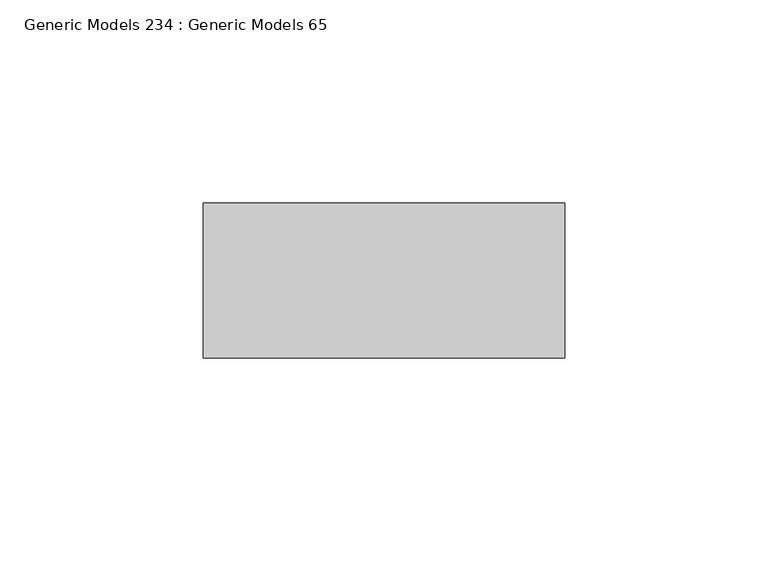
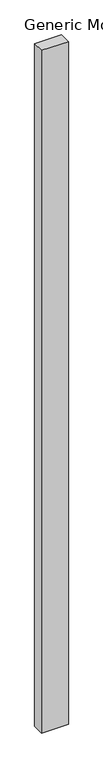
"""IFC4 building model written with IfcOpenShell, lengths in millimetres: proxy geometry, Generic Models 234 : Generic Models 65."""

import ifcopenshell
import ifcopenshell.guid

model = None  # the IFC model being written
_history = None  # IfcOwnerHistory: only IFC2X3 demands one
_inside = {}  # id of a spatial element -> (the spatial element, [elements in it])
_under = {}  # id of a project, library or spatial element -> (it, [spatial elements below it])
_declared = {}  # id of a project -> (the project, [libraries it declares])
_typed = {}  # id of a type object -> (the type object, [elements of that type])
_made_of = {}  # id of a material, layer set ... -> (it, [elements and type objects made of it])


def new_model(schema):
    """Start an empty IFC model of exactly this schema.

    Asked for "IFC4X3", IfcOpenShell would pick the latest addendum, in which some entities
    have other attributes; the version numbers below select the first issue.
    IFC2X3 requires an IfcOwnerHistory on every rooted entity: one is made here for all.
    """
    global model, _history
    if schema == "IFC4X3":
        model = ifcopenshell.file(schema_version=(4, 3, 0, 0))
    else:
        model = ifcopenshell.file(schema=schema)
    _inside.clear()
    _under.clear()
    _declared.clear()
    _typed.clear()
    _made_of.clear()
    _history = None
    if model.schema == "IFC2X3":
        org = make("IfcOrganization", Name="unknown")
        user = make(
            "IfcPersonAndOrganization",
            ThePerson=make("IfcPerson", FamilyName="unknown"),
            TheOrganization=org,
        )
        app = make(
            "IfcApplication",
            ApplicationDeveloper=org,
            Version="unknown",
            ApplicationFullName="unknown",
            ApplicationIdentifier="unknown",
        )
        _history = make(
            "IfcOwnerHistory",
            OwningUser=user,
            OwningApplication=app,
            ChangeAction="ADDED",
            CreationDate=0,
        )
    return model


def make(cls, **values):
    """One entity of the class cls with the attributes given. An attribute that is None is left unset."""
    return model.create_entity(
        cls, **{name: value for name, value in values.items() if value is not None}
    )


def rooted(cls, **values):
    """An entity with a GlobalId (a new one), such as an element, a storey or a relation."""
    return make(cls, GlobalId=ifcopenshell.guid.new(), OwnerHistory=_history, **values)


def si_unit(unit_type, name, prefix=None):
    """IfcSIUnit, for example si_unit("LENGTHUNIT", "METRE", prefix="MILLI")."""
    return make("IfcSIUnit", UnitType=unit_type, Prefix=prefix, Name=name)


def assignment(units):
    """IfcUnitAssignment: the units of a project."""
    return None if units is None else make("IfcUnitAssignment", Units=units)


def point(xyz):
    """IfcCartesianPoint."""
    return None if xyz is None else make("IfcCartesianPoint", Coordinates=xyz)


def direction(xyz):
    """IfcDirection."""
    return None if xyz is None else make("IfcDirection", DirectionRatios=xyz)


def frame(location, z_axis=None, x_axis=None):
    """IfcAxis2Placement3D, a coordinate frame: its origin and axes. An axis left out is left unset."""
    return make(
        "IfcAxis2Placement3D",
        Location=point(location),
        Axis=direction(z_axis),
        RefDirection=direction(x_axis),
    )


def origin():
    """The frame at (0, 0, 0) with its axes left unset."""
    return frame((0.0, 0.0, 0.0))


def place(relative_to, where):
    """IfcLocalPlacement: puts the frame where relative to a parent placement (None: the world)."""
    return make(
        "IfcLocalPlacement", PlacementRelTo=relative_to, RelativePlacement=where
    )


def context(
    kind, dimensions, precision=None, world=None, true_north=None, identifier=None
):
    """IfcGeometricRepresentationContext, for example the 3D "Model" context."""
    return make(
        "IfcGeometricRepresentationContext",
        ContextIdentifier=identifier,
        ContextType=kind,
        CoordinateSpaceDimension=dimensions,
        Precision=precision,
        WorldCoordinateSystem=world,
        TrueNorth=true_north,
    )


def project(units=None, contexts=None):
    """IfcProject with its units and contexts."""
    return rooted(
        "IfcProject",
        Name="project",
        RepresentationContexts=contexts,
        UnitsInContext=assignment(units),
    )


def spatial(cls, under=None, at=None, **own):
    """A site, building, storey or space (cls), placed at a placement, below another one or the project."""
    s = rooted(cls, ObjectPlacement=at, **own)
    if under is not None:
        _under.setdefault(under.id(), (under, []))[1].append(s)
    return s


def polyline(points):
    """IfcPolyline through the points."""
    return make("IfcPolyline", Points=[point(p) for p in points])


def outline(outer, holes=None, kind="AREA"):
    """IfcArbitraryClosedProfileDef: a profile drawn as a closed curve; with holes, ...WithVoids."""
    if holes is None:
        return make("IfcArbitraryClosedProfileDef", ProfileType=kind, OuterCurve=outer)
    return make(
        "IfcArbitraryProfileDefWithVoids",
        ProfileType=kind,
        OuterCurve=outer,
        InnerCurves=holes,
    )


def extrude(swept, where, along, depth):
    """IfcExtrudedAreaSolid: the profile swept, set in the frame where, extruded along a direction by depth."""
    return make(
        "IfcExtrudedAreaSolid",
        SweptArea=swept,
        Position=where,
        ExtrudedDirection=direction(along),
        Depth=depth,
    )


def shape(context_of_items, identifier, shape_type, items):
    """IfcShapeRepresentation: the items that make up one representation, for example the "Body"."""
    return make(
        "IfcShapeRepresentation",
        ContextOfItems=context_of_items,
        RepresentationIdentifier=identifier,
        RepresentationType=shape_type,
        Items=items,
    )


def source(mapping_origin, context_of_items, identifier, shape_type, items):
    """IfcRepresentationMap: a shape defined once, which mapped items show again and again."""
    return make(
        "IfcRepresentationMap",
        MappingOrigin=mapping_origin,
        MappedRepresentation=shape(context_of_items, identifier, shape_type, items),
    )


def transform(
    local_origin,
    x_axis=None,
    y_axis=None,
    z_axis=None,
    scale=None,
    scale2=None,
    scale3=None,
    uniform=True,
):
    """IfcCartesianTransformationOperator3D, or its non-uniform kind. x_axis, y_axis, z_axis: its Axis1, 2, 3."""
    if uniform:
        return make(
            "IfcCartesianTransformationOperator3D",
            Axis1=direction(x_axis),
            Axis2=direction(y_axis),
            LocalOrigin=point(local_origin),
            Scale=scale,
            Axis3=direction(z_axis),
        )
    return make(
        "IfcCartesianTransformationOperator3DnonUniform",
        Axis1=direction(x_axis),
        Axis2=direction(y_axis),
        LocalOrigin=point(local_origin),
        Scale=scale,
        Axis3=direction(z_axis),
        Scale2=scale2,
        Scale3=scale3,
    )


def mapped(mapping_source, mapping_target):
    """IfcMappedItem: shows the shape of a source again, moved by a transform."""
    return make(
        "IfcMappedItem", MappingSource=mapping_source, MappingTarget=mapping_target
    )


def made_of(thing, what):
    """Note that an element or type object is made of a material, layer set ...; save() writes the relation."""
    if what is not None:
        _made_of.setdefault(what.id(), (what, []))[1].append(thing)
    return thing


def element(
    cls,
    number,
    at=None,
    inside=None,
    cuts=None,
    type_object=None,
    material=None,
    context=None,
    identifier="Body",
    shape_type=None,
    held_by="IfcProductDefinitionShape",
    body=None,
    shapes=None,
    **own,
):
    """One element of the class cls, such as IfcWall. Its Tag is "e" and its number.

    at: its placement. inside: the storey or other place that contains it. cuts: it is an
    opening in that element (IfcRelVoidsElement). A single representation is given by context,
    identifier, shape_type and body (its items); several are given by shapes. held_by: the class
    of the entity that holds the representations. save() writes the other relations.
    """
    e = rooted(cls, Tag="e%d" % number, ObjectPlacement=at, **own)
    if body is not None:
        shapes = [shape(context, identifier, shape_type, body)]
    if shapes is not None:
        e.Representation = make(held_by, Representations=shapes)
    if inside is not None:
        _inside.setdefault(inside.id(), (inside, []))[1].append(e)
    if cuts is not None:
        rooted(
            "IfcRelVoidsElement", RelatingBuildingElement=cuts, RelatedOpeningElement=e
        )
    if type_object is not None:
        _typed.setdefault(type_object.id(), (type_object, []))[1].append(e)
    return made_of(e, material)


def aggregate(whole, parts):
    """IfcRelAggregates: a whole, such as a stair, and the parts it consists of."""
    return rooted("IfcRelAggregates", RelatingObject=whole, RelatedObjects=parts)


def save(model, path):
    """Write the relations noted so far, then the file.

    IfcRelAggregates (storeys below a building ...), IfcRelContainedInSpatialStructure (elements
    in a storey), IfcRelDefinesByType, IfcRelAssociatesMaterial and IfcRelDeclares: one each for
    every whole, place, type object, material and project.
    """
    for whole, parts in _under.values():
        aggregate(whole, parts)
    for where, things in _inside.values():
        rooted(
            "IfcRelContainedInSpatialStructure",
            RelatedElements=things,
            RelatingStructure=where,
        )
    for kind, things in _typed.values():
        rooted("IfcRelDefinesByType", RelatedObjects=things, RelatingType=kind)
    for what, things in _made_of.values():
        rooted("IfcRelAssociatesMaterial", RelatedObjects=things, RelatingMaterial=what)
    for by, libraries in _declared.values():
        rooted("IfcRelDeclares", RelatingContext=by, RelatedDefinitions=libraries)
    model.write(path)


def generic_models_234_generic_models_65_886ed74c(model_context):
    return source(origin(), model_context, "Body", "SweptSolid", [
        extrude(outline(polyline([(49784.0, 592.1375), (49695.1, 592.1375), (49695.1, 630.2375), (49784.0, 630.2375), (49784.0, 592.1375)])), frame((0.0, 0.0, 3086.1), z_axis=(0.0, 0.0, 1.0), x_axis=(1.0, 0.0, 0.0)), (0.0, 0.0, 1.0), 2381.25),
    ])


if __name__ == "__main__":
    model = new_model("IFC4")
    model_context = context("Model", 3, world=origin())
    ifc_project = project(units=[si_unit("LENGTHUNIT", "METRE", prefix="MILLI")], contexts=[model_context])
    site = spatial("IfcSite", under=ifc_project)
    building = spatial("IfcBuilding", under=site)
    placement = place(None, origin())
    generic_models_234_generic_models_65_shape = generic_models_234_generic_models_65_886ed74c(model_context)
    element("IfcBuildingElementProxy", 1, Name="Generic Models 234 : Generic Models 65", ObjectType="Generic Models 234 : Generic Models 65", at=placement, inside=building, context=model_context, shape_type="MappedRepresentation", body=[
        mapped(generic_models_234_generic_models_65_shape, transform((0.0, 0.0, 0.0), x_axis=(1.0, 0.0, 0.0), y_axis=(0.0, 1.0, 0.0), z_axis=(0.0, 0.0, 1.0))),
    ])
    save(model, "model.ifc")

# Revit data of these elements
# Element 1 (IfcBuildingElementProxy, "Generic Models 234 : Generic Models 65")
#   Materials on its faces: "2X WOOD STUD - SEE 'WALL TAG' & 'LAYER MATERIAL SCHEDULE' FOR SPACING & INSULATION TREATMENT, IF APPLICAPLE"
# Materials
#   "2X WOOD STUD - SEE 'WALL TAG' & 'LAYER MATERIAL SCHEDULE' FOR SPACING & INSULATION TREATMENT, IF APPLICAPLE": class "Wood", colour RGB 234 198 147, transparency 0, Description = "Pinus Echinata", Cost = 0
